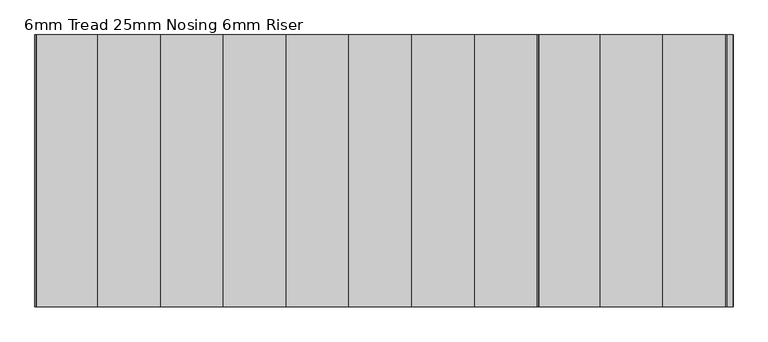
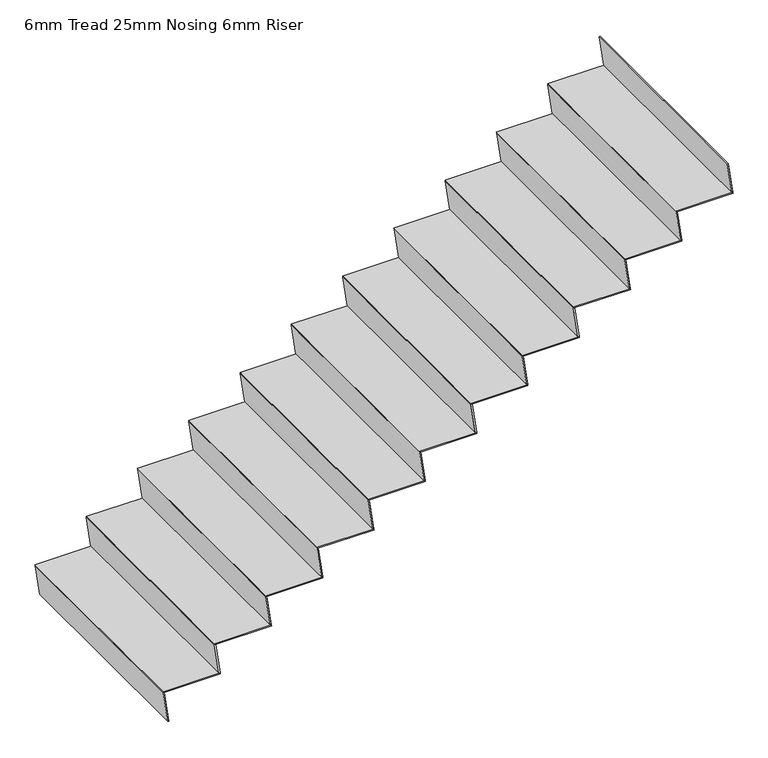
"""IFC4 building model written with IfcOpenShell, lengths in millimetres: stair flight geometry, 6mm Tread 25mm Nosing 6mm Riser."""

from ifc_helpers import new_model, si_unit, origin, place, context, project, spatial, faceted_brep, source, transform, mapped, element, save


def stair_flight_6mm_tread_25mm_nosing_6mm_riser_f88628f3(model_context):
    return source(origin(), model_context, "Body", "Brep", [
        faceted_brep([(-16043.9400908, 12030.4345331, 14352.9411765), (-16043.0900908, 12030.4345331, 14346.9411765), (-16043.0900908, 13220.4345331, 14346.9411765), (-16043.9400908, 13220.4345331, 14352.9411765), (-16350.0, 13220.4345331, 14352.9411765), (-16350.0, 12030.4345331, 14352.9411765), (-16349.15, 12030.4345331, 14346.9411765), (-16349.15, 13220.4345331, 14346.9411765)], [[[0, 1, 2, 3]], [[3, 4, 5, 0]], [[2, 1, 6, 7]], [[4, 3, 2, 7]], [[0, 5, 6, 1]], [[5, 4, 7, 6]]]),
        faceted_brep([(-16349.15, 12030.4345331, 14346.9411765), (-16325.0, 12030.4345331, 14176.4705882), (-16318.9400908, 12030.4345331, 14176.4705882), (-16343.0900908, 12030.4345331, 14346.9411765), (-16349.15, 13220.4345331, 14346.9411765), (-16343.0900908, 13220.4345331, 14346.9411765), (-16318.9400908, 13220.4345331, 14176.4705882), (-16325.0, 13220.4345331, 14176.4705882)], [[[0, 1, 2, 3]], [[4, 5, 6, 7]], [[1, 0, 4, 7]], [[2, 1, 7, 6]], [[3, 2, 6, 5]], [[0, 3, 5, 4]]]),
        faceted_brep([(-16074.15, 12030.4345331, 14523.4117647), (-16050.0, 12030.4345331, 14352.9411765), (-16043.9400908, 12030.4345331, 14352.9411765), (-16068.0900908, 12030.4345331, 14523.4117647), (-16074.15, 13220.4345331, 14523.4117647), (-16068.0900908, 13220.4345331, 14523.4117647), (-16043.9400908, 13220.4345331, 14352.9411765), (-16050.0, 13220.4345331, 14352.9411765)], [[[0, 1, 2, 3]], [[4, 5, 6, 7]], [[1, 0, 4, 7]], [[2, 1, 7, 6]], [[3, 2, 6, 5]], [[0, 3, 5, 4]]]),
        faceted_brep([(-15768.9400908, 13220.4345331, 14529.4117647), (-16075.0, 13220.4345331, 14529.4117647), (-16075.0, 12030.4345331, 14529.4117647), (-15768.9400908, 12030.4345331, 14529.4117647), (-15768.0900908, 13220.4345331, 14523.4117647), (-15768.0900908, 12030.4345331, 14523.4117647), (-16074.15, 12030.4345331, 14523.4117647), (-16074.15, 13220.4345331, 14523.4117647)], [[[0, 1, 2, 3]], [[4, 5, 6, 7]], [[1, 0, 4, 7]], [[3, 2, 6, 5]], [[3, 5, 4, 0]], [[2, 1, 7, 6]]]),
        faceted_brep([(-15799.15, 12030.4345331, 14699.8823529), (-15775.0, 12030.4345331, 14529.4117647), (-15768.9400908, 12030.4345331, 14529.4117647), (-15793.0900908, 12030.4345331, 14699.8823529), (-15799.15, 13220.4345331, 14699.8823529), (-15793.0900908, 13220.4345331, 14699.8823529), (-15768.9400908, 13220.4345331, 14529.4117647), (-15775.0, 13220.4345331, 14529.4117647)], [[[0, 1, 2, 3]], [[4, 5, 6, 7]], [[1, 0, 4, 7]], [[2, 1, 7, 6]], [[3, 2, 6, 5]], [[0, 3, 5, 4]]]),
        faceted_brep([(-15493.9400908, 13220.4345331, 14705.8823529), (-15800.0, 13220.4345331, 14705.8823529), (-15800.0, 12030.4345331, 14705.8823529), (-15493.9400908, 12030.4345331, 14705.8823529), (-15493.0900908, 13220.4345331, 14699.8823529), (-15493.0900908, 12030.4345331, 14699.8823529), (-15799.15, 12030.4345331, 14699.8823529), (-15799.15, 13220.4345331, 14699.8823529)], [[[0, 1, 2, 3]], [[4, 5, 6, 7]], [[1, 0, 4, 7]], [[3, 2, 6, 5]], [[3, 5, 4, 0]], [[2, 1, 7, 6]]]),
        faceted_brep([(-15524.15, 12030.4345331, 14876.3529412), (-15500.0, 12030.4345331, 14705.8823529), (-15493.9400908, 12030.4345331, 14705.8823529), (-15518.0900908, 12030.4345331, 14876.3529412), (-15524.15, 13220.4345331, 14876.3529412), (-15518.0900908, 13220.4345331, 14876.3529412), (-15493.9400908, 13220.4345331, 14705.8823529), (-15500.0, 13220.4345331, 14705.8823529)], [[[0, 1, 2, 3]], [[4, 5, 6, 7]], [[1, 0, 4, 7]], [[2, 1, 7, 6]], [[3, 2, 6, 5]], [[0, 3, 5, 4]]]),
        faceted_brep([(-15218.9400908, 13220.4345331, 14882.3529412), (-15525.0, 13220.4345331, 14882.3529412), (-15525.0, 12030.4345331, 14882.3529412), (-15218.9400908, 12030.4345331, 14882.3529412), (-15218.0900908, 13220.4345331, 14876.3529412), (-15218.0900908, 12030.4345331, 14876.3529412), (-15524.15, 12030.4345331, 14876.3529412), (-15524.15, 13220.4345331, 14876.3529412)], [[[0, 1, 2, 3]], [[4, 5, 6, 7]], [[1, 0, 4, 7]], [[3, 2, 6, 5]], [[3, 5, 4, 0]], [[2, 1, 7, 6]]]),
        faceted_brep([(-15249.15, 12030.4345331, 15052.8235294), (-15225.0, 12030.4345331, 14882.3529412), (-15218.9400908, 12030.4345331, 14882.3529412), (-15243.0900908, 12030.4345331, 15052.8235294), (-15249.15, 13220.4345331, 15052.8235294), (-15243.0900908, 13220.4345331, 15052.8235294), (-15218.9400908, 13220.4345331, 14882.3529412), (-15225.0, 13220.4345331, 14882.3529412)], [[[0, 1, 2, 3]], [[4, 5, 6, 7]], [[1, 0, 4, 7]], [[2, 1, 7, 6]], [[3, 2, 6, 5]], [[0, 3, 5, 4]]]),
        faceted_brep([(-14943.9400908, 13220.4345331, 15058.8235294), (-15250.0, 13220.4345331, 15058.8235294), (-15250.0, 12030.4345331, 15058.8235294), (-14943.9400908, 12030.4345331, 15058.8235294), (-14943.0900908, 13220.4345331, 15052.8235294), (-14943.0900908, 12030.4345331, 15052.8235294), (-15249.15, 12030.4345331, 15052.8235294), (-15249.15, 13220.4345331, 15052.8235294)], [[[0, 1, 2, 3]], [[4, 5, 6, 7]], [[1, 0, 4, 7]], [[3, 2, 6, 5]], [[3, 5, 4, 0]], [[2, 1, 7, 6]]]),
        faceted_brep([(-14974.15, 12030.4345331, 15229.2941176), (-14950.0, 12030.4345331, 15058.8235294), (-14943.9400908, 12030.4345331, 15058.8235294), (-14968.0900908, 12030.4345331, 15229.2941176), (-14974.15, 13220.4345331, 15229.2941176), (-14968.0900908, 13220.4345331, 15229.2941176), (-14943.9400908, 13220.4345331, 15058.8235294), (-14950.0, 13220.4345331, 15058.8235294)], [[[0, 1, 2, 3]], [[4, 5, 6, 7]], [[1, 0, 4, 7]], [[2, 1, 7, 6]], [[3, 2, 6, 5]], [[0, 3, 5, 4]]]),
        faceted_brep([(-14668.9400908, 13220.4345331, 15235.2941176), (-14975.0, 13220.4345331, 15235.2941176), (-14975.0, 12030.4345331, 15235.2941176), (-14668.9400908, 12030.4345331, 15235.2941176), (-14668.0900908, 13220.4345331, 15229.2941176), (-14668.0900908, 12030.4345331, 15229.2941176), (-14974.15, 12030.4345331, 15229.2941176), (-14974.15, 13220.4345331, 15229.2941176)], [[[0, 1, 2, 3]], [[4, 5, 6, 7]], [[1, 0, 4, 7]], [[3, 2, 6, 5]], [[3, 5, 4, 0]], [[2, 1, 7, 6]]]),
        faceted_brep([(-14699.15, 12030.4345331, 15405.7647059), (-14675.0, 12030.4345331, 15235.2941176), (-14668.9400908, 12030.4345331, 15235.2941176), (-14693.0900908, 12030.4345331, 15405.7647059), (-14699.15, 13220.4345331, 15405.7647059), (-14693.0900908, 13220.4345331, 15405.7647059), (-14668.9400908, 13220.4345331, 15235.2941176), (-14675.0, 13220.4345331, 15235.2941176)], [[[0, 1, 2, 3]], [[4, 5, 6, 7]], [[1, 0, 4, 7]], [[2, 1, 7, 6]], [[3, 2, 6, 5]], [[0, 3, 5, 4]]]),
        faceted_brep([(-14393.9400908, 13220.4345331, 15411.7647059), (-14700.0, 13220.4345331, 15411.7647059), (-14700.0, 12030.4345331, 15411.7647059), (-14393.9400908, 12030.4345331, 15411.7647059), (-14393.0900908, 13220.4345331, 15405.7647059), (-14393.0900908, 12030.4345331, 15405.7647059), (-14699.15, 12030.4345331, 15405.7647059), (-14699.15, 13220.4345331, 15405.7647059)], [[[0, 1, 2, 3]], [[4, 5, 6, 7]], [[1, 0, 4, 7]], [[3, 2, 6, 5]], [[3, 5, 4, 0]], [[2, 1, 7, 6]]]),
        faceted_brep([(-14424.15, 12030.4345331, 15582.2352941), (-14400.0, 12030.4345331, 15411.7647059), (-14393.9400908, 12030.4345331, 15411.7647059), (-14418.0900908, 12030.4345331, 15582.2352941), (-14424.15, 13220.4345331, 15582.2352941), (-14418.0900908, 13220.4345331, 15582.2352941), (-14393.9400908, 13220.4345331, 15411.7647059), (-14400.0, 13220.4345331, 15411.7647059)], [[[0, 1, 2, 3]], [[4, 5, 6, 7]], [[1, 0, 4, 7]], [[2, 1, 7, 6]], [[3, 2, 6, 5]], [[0, 3, 5, 4]]]),
        faceted_brep([(-14118.9400908, 13220.4345331, 15588.2352941), (-14425.0, 13220.4345331, 15588.2352941), (-14425.0, 12030.4345331, 15588.2352941), (-14118.9400908, 12030.4345331, 15588.2352941), (-14118.0900908, 13220.4345331, 15582.2352941), (-14118.0900908, 12030.4345331, 15582.2352941), (-14424.15, 12030.4345331, 15582.2352941), (-14424.15, 13220.4345331, 15582.2352941)], [[[0, 1, 2, 3]], [[4, 5, 6, 7]], [[1, 0, 4, 7]], [[3, 2, 6, 5]], [[3, 5, 4, 0]], [[2, 1, 7, 6]]]),
        faceted_brep([(-14149.15, 12030.4345331, 15758.7058824), (-14125.0, 12030.4345331, 15588.2352941), (-14118.9400908, 12030.4345331, 15588.2352941), (-14143.0900908, 12030.4345331, 15758.7058824), (-14149.15, 13220.4345331, 15758.7058824), (-14143.0900908, 13220.4345331, 15758.7058824), (-14118.9400908, 13220.4345331, 15588.2352941), (-14125.0, 13220.4345331, 15588.2352941)], [[[0, 1, 2, 3]], [[4, 5, 6, 7]], [[1, 0, 4, 7]], [[2, 1, 7, 6]], [[3, 2, 6, 5]], [[0, 3, 5, 4]]]),
        faceted_brep([(-13843.9400908, 13220.4345331, 15764.7058824), (-14150.0, 13220.4345331, 15764.7058824), (-14150.0, 12030.4345331, 15764.7058824), (-13843.9400908, 12030.4345331, 15764.7058824), (-13843.0900908, 13220.4345331, 15758.7058824), (-13843.0900908, 12030.4345331, 15758.7058824), (-14149.15, 12030.4345331, 15758.7058824), (-14149.15, 13220.4345331, 15758.7058824)], [[[0, 1, 2, 3]], [[4, 5, 6, 7]], [[1, 0, 4, 7]], [[3, 2, 6, 5]], [[3, 5, 4, 0]], [[2, 1, 7, 6]]]),
        faceted_brep([(-13874.15, 12030.4345331, 15935.1764706), (-13850.0, 12030.4345331, 15764.7058824), (-13843.9400908, 12030.4345331, 15764.7058824), (-13868.0900908, 12030.4345331, 15935.1764706), (-13874.15, 13220.4345331, 15935.1764706), (-13868.0900908, 13220.4345331, 15935.1764706), (-13843.9400908, 13220.4345331, 15764.7058824), (-13850.0, 13220.4345331, 15764.7058824)], [[[0, 1, 2, 3]], [[4, 5, 6, 7]], [[1, 0, 4, 7]], [[2, 1, 7, 6]], [[3, 2, 6, 5]], [[0, 3, 5, 4]]]),
        faceted_brep([(-13568.9400908, 13220.4345331, 15941.1764706), (-13875.0, 13220.4345331, 15941.1764706), (-13875.0, 12030.4345331, 15941.1764706), (-13568.9400908, 12030.4345331, 15941.1764706), (-13568.0900908, 13220.4345331, 15935.1764706), (-13568.0900908, 12030.4345331, 15935.1764706), (-13874.15, 12030.4345331, 15935.1764706), (-13874.15, 13220.4345331, 15935.1764706)], [[[0, 1, 2, 3]], [[4, 5, 6, 7]], [[1, 0, 4, 7]], [[3, 2, 6, 5]], [[3, 5, 4, 0]], [[2, 1, 7, 6]]]),
        faceted_brep([(-13324.15, 12030.4345331, 16288.1176471), (-13300.0, 12030.4345331, 16117.6470588), (-13293.9400908, 12030.4345331, 16117.6470588), (-13318.0900908, 12030.4345331, 16288.1176471), (-13324.15, 13220.4345331, 16288.1176471), (-13318.0900908, 13220.4345331, 16288.1176471), (-13293.9400908, 13220.4345331, 16117.6470588), (-13300.0, 13220.4345331, 16117.6470588)], [[[0, 1, 2, 3]], [[4, 5, 6, 7]], [[1, 0, 4, 7]], [[2, 1, 7, 6]], [[3, 2, 6, 5]], [[0, 3, 5, 4]]]),
        faceted_brep([(-13599.15, 12030.4345331, 16111.6470588), (-13575.0, 12030.4345331, 15941.1764706), (-13568.9400908, 12030.4345331, 15941.1764706), (-13593.0900908, 12030.4345331, 16111.6470588), (-13599.15, 13220.4345331, 16111.6470588), (-13593.0900908, 13220.4345331, 16111.6470588), (-13568.9400908, 13220.4345331, 15941.1764706), (-13575.0, 13220.4345331, 15941.1764706)], [[[0, 1, 2, 3]], [[4, 5, 6, 7]], [[1, 0, 4, 7]], [[2, 1, 7, 6]], [[3, 2, 6, 5]], [[0, 3, 5, 4]]]),
        faceted_brep([(-13293.9400908, 13220.4345331, 16117.6470588), (-13325.0, 13220.4345331, 16117.6470588), (-13600.0, 13220.4345331, 16117.6470588), (-13600.0, 12030.4345331, 16117.6470588), (-13293.9400908, 12030.4345331, 16117.6470588), (-13293.0900908, 13220.4345331, 16111.6470588), (-13293.0900908, 12030.4345331, 16111.6470588), (-13599.15, 12030.4345331, 16111.6470588), (-13599.15, 13220.4345331, 16111.6470588), (-13325.0, 13220.4345331, 16111.6470588)], [[[0, 1, 2, 3, 4]], [[5, 6, 7, 8, 9]], [[1, 0, 5, 9]], [[2, 1, 9, 8]], [[4, 3, 7, 6]], [[4, 6, 5, 0]], [[3, 2, 8, 7]]]),
    ])


if __name__ == "__main__":
    model = new_model("IFC4")
    model_context = context("Model", 3, world=origin())
    ifc_project = project(units=[si_unit("LENGTHUNIT", "METRE", prefix="MILLI")], contexts=[model_context])
    site = spatial("IfcSite", under=ifc_project)
    building = spatial("IfcBuilding", under=site)
    placement = place(None, origin())
    stair_flight_6mm_tread_25mm_nosing_6mm_riser_shape = stair_flight_6mm_tread_25mm_nosing_6mm_riser_f88628f3(model_context)
    element("IfcStairFlight", 1, ObjectType="6mm Tread 25mm Nosing 6mm Riser", at=placement, inside=building, context=model_context, shape_type="MappedRepresentation", body=[
        mapped(stair_flight_6mm_tread_25mm_nosing_6mm_riser_shape, transform((0.0, 0.0, 0.0), x_axis=(1.0, 0.0, 0.0), y_axis=(0.0, 1.0, 0.0), z_axis=(0.0, 0.0, 1.0))),
    ])
    save(model, "model.ifc")

# Revit data of these elements
# Element 1 (IfcStairFlight, "6mm Tread 25mm Nosing 6mm Riser")
#   Materials on its faces: "Steel, Paint Finish, Dark Gray"
# Materials
#   "Steel, Paint Finish, Dark Gray": class "Metal", colour RGB 89 89 89, transparency 0, Description = "Steel, paint finish, dark gray, glossy", Cost = 0
